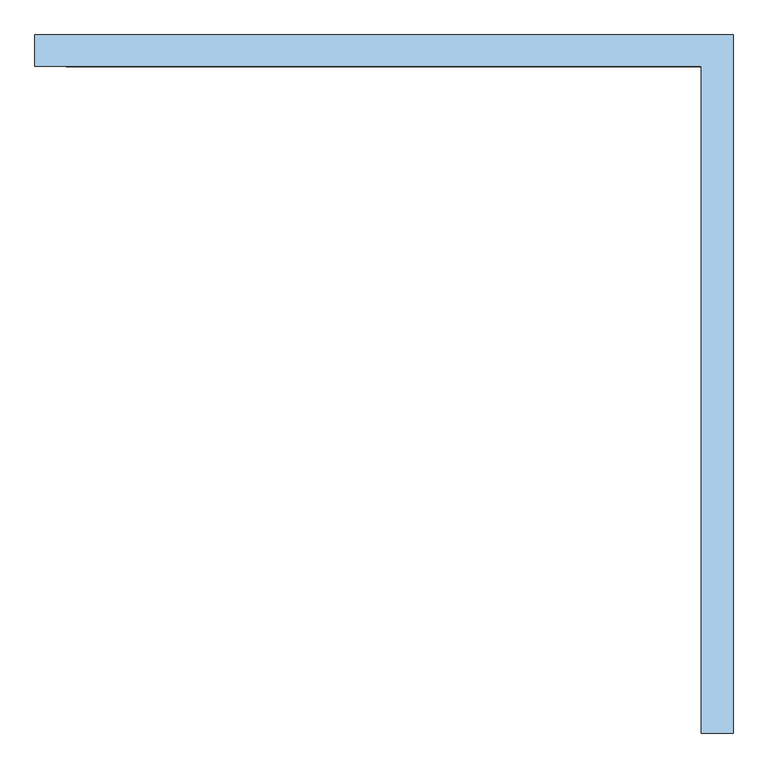
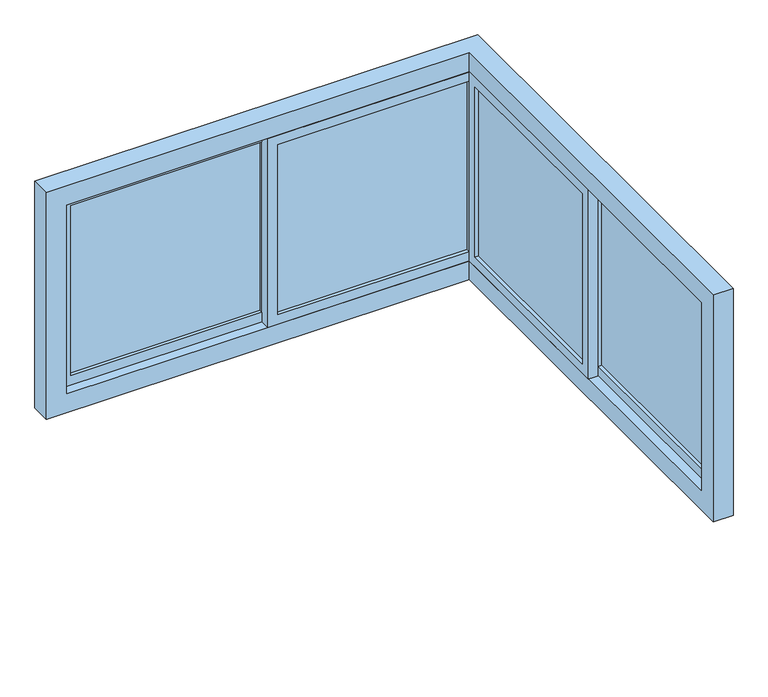
"""IFC4 building model written with IfcOpenShell, lengths in millimetres: window geometry, .CC_ND 300_JANELA DE CANTO_4 FOLHAS DE CORRER_VIDRO : 1.20F X 1.20E X 0.60H."""

import ifcopenshell
import ifcopenshell.guid

model = None  # the IFC model being written
_history = None  # IfcOwnerHistory: only IFC2X3 demands one
_inside = {}  # id of a spatial element -> (the spatial element, [elements in it])
_under = {}  # id of a project, library or spatial element -> (it, [spatial elements below it])
_declared = {}  # id of a project -> (the project, [libraries it declares])
_typed = {}  # id of a type object -> (the type object, [elements of that type])
_made_of = {}  # id of a material, layer set ... -> (it, [elements and type objects made of it])


def new_model(schema):
    """Start an empty IFC model of exactly this schema.

    Asked for "IFC4X3", IfcOpenShell would pick the latest addendum, in which some entities
    have other attributes; the version numbers below select the first issue.
    IFC2X3 requires an IfcOwnerHistory on every rooted entity: one is made here for all.
    """
    global model, _history
    if schema == "IFC4X3":
        model = ifcopenshell.file(schema_version=(4, 3, 0, 0))
    else:
        model = ifcopenshell.file(schema=schema)
    _inside.clear()
    _under.clear()
    _declared.clear()
    _typed.clear()
    _made_of.clear()
    _history = None
    if model.schema == "IFC2X3":
        org = make("IfcOrganization", Name="unknown")
        user = make(
            "IfcPersonAndOrganization",
            ThePerson=make("IfcPerson", FamilyName="unknown"),
            TheOrganization=org,
        )
        app = make(
            "IfcApplication",
            ApplicationDeveloper=org,
            Version="unknown",
            ApplicationFullName="unknown",
            ApplicationIdentifier="unknown",
        )
        _history = make(
            "IfcOwnerHistory",
            OwningUser=user,
            OwningApplication=app,
            ChangeAction="ADDED",
            CreationDate=0,
        )
    return model


def make(cls, **values):
    """One entity of the class cls with the attributes given. An attribute that is None is left unset."""
    return model.create_entity(
        cls, **{name: value for name, value in values.items() if value is not None}
    )


def rooted(cls, **values):
    """An entity with a GlobalId (a new one), such as an element, a storey or a relation."""
    return make(cls, GlobalId=ifcopenshell.guid.new(), OwnerHistory=_history, **values)


def si_unit(unit_type, name, prefix=None):
    """IfcSIUnit, for example si_unit("LENGTHUNIT", "METRE", prefix="MILLI")."""
    return make("IfcSIUnit", UnitType=unit_type, Prefix=prefix, Name=name)


def assignment(units):
    """IfcUnitAssignment: the units of a project."""
    return None if units is None else make("IfcUnitAssignment", Units=units)


def point(xyz):
    """IfcCartesianPoint."""
    return None if xyz is None else make("IfcCartesianPoint", Coordinates=xyz)


def direction(xyz):
    """IfcDirection."""
    return None if xyz is None else make("IfcDirection", DirectionRatios=xyz)


def frame(location, z_axis=None, x_axis=None):
    """IfcAxis2Placement3D, a coordinate frame: its origin and axes. An axis left out is left unset."""
    return make(
        "IfcAxis2Placement3D",
        Location=point(location),
        Axis=direction(z_axis),
        RefDirection=direction(x_axis),
    )


def origin():
    """The frame at (0, 0, 0) with its axes left unset."""
    return frame((0.0, 0.0, 0.0))


def place(relative_to, where):
    """IfcLocalPlacement: puts the frame where relative to a parent placement (None: the world)."""
    return make(
        "IfcLocalPlacement", PlacementRelTo=relative_to, RelativePlacement=where
    )


def context(
    kind, dimensions, precision=None, world=None, true_north=None, identifier=None
):
    """IfcGeometricRepresentationContext, for example the 3D "Model" context."""
    return make(
        "IfcGeometricRepresentationContext",
        ContextIdentifier=identifier,
        ContextType=kind,
        CoordinateSpaceDimension=dimensions,
        Precision=precision,
        WorldCoordinateSystem=world,
        TrueNorth=true_north,
    )


def project(units=None, contexts=None):
    """IfcProject with its units and contexts."""
    return rooted(
        "IfcProject",
        Name="project",
        RepresentationContexts=contexts,
        UnitsInContext=assignment(units),
    )


def spatial(cls, under=None, at=None, **own):
    """A site, building, storey or space (cls), placed at a placement, below another one or the project."""
    s = rooted(cls, ObjectPlacement=at, **own)
    if under is not None:
        _under.setdefault(under.id(), (under, []))[1].append(s)
    return s


def polyline(points):
    """IfcPolyline through the points."""
    return make("IfcPolyline", Points=[point(p) for p in points])


def outline(outer, holes=None, kind="AREA"):
    """IfcArbitraryClosedProfileDef: a profile drawn as a closed curve; with holes, ...WithVoids."""
    if holes is None:
        return make("IfcArbitraryClosedProfileDef", ProfileType=kind, OuterCurve=outer)
    return make(
        "IfcArbitraryProfileDefWithVoids",
        ProfileType=kind,
        OuterCurve=outer,
        InnerCurves=holes,
    )


def extrude(swept, where, along, depth):
    """IfcExtrudedAreaSolid: the profile swept, set in the frame where, extruded along a direction by depth."""
    return make(
        "IfcExtrudedAreaSolid",
        SweptArea=swept,
        Position=where,
        ExtrudedDirection=direction(along),
        Depth=depth,
    )


def faces_of(points, faces, orient=None, outer=None):
    """IfcFace entities. A face is a list of loops; a loop is a list of indices into points, from 0.

    orient and outer hold one flag for each loop. By default every Orientation is true, the
    first loop of a face is its IfcFaceOuterBound and the others are IfcFaceBound.
    """
    made = []
    for i, loops in enumerate(faces):
        bounds = []
        for j, loop in enumerate(loops):
            is_outer = j == 0 if outer is None else outer[i][j]
            bounds.append(
                make(
                    "IfcFaceOuterBound" if is_outer else "IfcFaceBound",
                    Bound=make("IfcPolyLoop", Polygon=[points[k] for k in loop]),
                    Orientation=True if orient is None else orient[i][j],
                )
            )
        made.append(make("IfcFace", Bounds=bounds))
    return made


def faceted_brep(points, faces, orient=None, outer=None, voids=None):
    """IfcFacetedBrep: a solid bounded by flat faces; with voids (closed shells), ...WithVoids."""
    shared = [point(p) for p in points]
    hull = make("IfcClosedShell", CfsFaces=faces_of(shared, faces, orient, outer))
    if voids is None:
        return make("IfcFacetedBrep", Outer=hull)
    return make(
        "IfcFacetedBrepWithVoids",
        Outer=hull,
        Voids=[
            make(cls, CfsFaces=faces_of(shared, fs, o, b)) for cls, fs, o, b in voids
        ],
    )


def shape(context_of_items, identifier, shape_type, items):
    """IfcShapeRepresentation: the items that make up one representation, for example the "Body"."""
    return make(
        "IfcShapeRepresentation",
        ContextOfItems=context_of_items,
        RepresentationIdentifier=identifier,
        RepresentationType=shape_type,
        Items=items,
    )


def source(mapping_origin, context_of_items, identifier, shape_type, items):
    """IfcRepresentationMap: a shape defined once, which mapped items show again and again."""
    return make(
        "IfcRepresentationMap",
        MappingOrigin=mapping_origin,
        MappedRepresentation=shape(context_of_items, identifier, shape_type, items),
    )


def transform(
    local_origin,
    x_axis=None,
    y_axis=None,
    z_axis=None,
    scale=None,
    scale2=None,
    scale3=None,
    uniform=True,
):
    """IfcCartesianTransformationOperator3D, or its non-uniform kind. x_axis, y_axis, z_axis: its Axis1, 2, 3."""
    if uniform:
        return make(
            "IfcCartesianTransformationOperator3D",
            Axis1=direction(x_axis),
            Axis2=direction(y_axis),
            LocalOrigin=point(local_origin),
            Scale=scale,
            Axis3=direction(z_axis),
        )
    return make(
        "IfcCartesianTransformationOperator3DnonUniform",
        Axis1=direction(x_axis),
        Axis2=direction(y_axis),
        LocalOrigin=point(local_origin),
        Scale=scale,
        Axis3=direction(z_axis),
        Scale2=scale2,
        Scale3=scale3,
    )


def mapped(mapping_source, mapping_target):
    """IfcMappedItem: shows the shape of a source again, moved by a transform."""
    return make(
        "IfcMappedItem", MappingSource=mapping_source, MappingTarget=mapping_target
    )


def made_of(thing, what):
    """Note that an element or type object is made of a material, layer set ...; save() writes the relation."""
    if what is not None:
        _made_of.setdefault(what.id(), (what, []))[1].append(thing)
    return thing


def element(
    cls,
    number,
    at=None,
    inside=None,
    cuts=None,
    type_object=None,
    material=None,
    context=None,
    identifier="Body",
    shape_type=None,
    held_by="IfcProductDefinitionShape",
    body=None,
    shapes=None,
    **own,
):
    """One element of the class cls, such as IfcWall. Its Tag is "e" and its number.

    at: its placement. inside: the storey or other place that contains it. cuts: it is an
    opening in that element (IfcRelVoidsElement). A single representation is given by context,
    identifier, shape_type and body (its items); several are given by shapes. held_by: the class
    of the entity that holds the representations. save() writes the other relations.
    """
    e = rooted(cls, Tag="e%d" % number, ObjectPlacement=at, **own)
    if body is not None:
        shapes = [shape(context, identifier, shape_type, body)]
    if shapes is not None:
        e.Representation = make(held_by, Representations=shapes)
    if inside is not None:
        _inside.setdefault(inside.id(), (inside, []))[1].append(e)
    if cuts is not None:
        rooted(
            "IfcRelVoidsElement", RelatingBuildingElement=cuts, RelatedOpeningElement=e
        )
    if type_object is not None:
        _typed.setdefault(type_object.id(), (type_object, []))[1].append(e)
    return made_of(e, material)


def aggregate(whole, parts):
    """IfcRelAggregates: a whole, such as a stair, and the parts it consists of."""
    return rooted("IfcRelAggregates", RelatingObject=whole, RelatedObjects=parts)


def save(model, path):
    """Write the relations noted so far, then the file.

    IfcRelAggregates (storeys below a building ...), IfcRelContainedInSpatialStructure (elements
    in a storey), IfcRelDefinesByType, IfcRelAssociatesMaterial and IfcRelDeclares: one each for
    every whole, place, type object, material and project.
    """
    for whole, parts in _under.values():
        aggregate(whole, parts)
    for where, things in _inside.values():
        rooted(
            "IfcRelContainedInSpatialStructure",
            RelatedElements=things,
            RelatingStructure=where,
        )
    for kind, things in _typed.values():
        rooted("IfcRelDefinesByType", RelatedObjects=things, RelatingType=kind)
    for what, things in _made_of.values():
        rooted("IfcRelAssociatesMaterial", RelatedObjects=things, RelatingMaterial=what)
    for by, libraries in _declared.values():
        rooted("IfcRelDeclares", RelatingContext=by, RelatedDefinitions=libraries)
    model.write(path)


def window_65d6727e(model_context):
    return source(origin(), model_context, "Body", "SolidModel", [
        extrude(outline(polyline([(-516.0, 1950.0), (-516.0, 1450.0), (-1032.0, 1450.0), (-1032.0, 1950.0), (-516.0, 1950.0)]), holes=[polyline([(-541.0, 1925.0), (-1007.0, 1925.0), (-1007.0, 1475.0), (-541.0, 1475.0), (-541.0, 1925.0)])]), frame((482.0, 0.0, 0.0), z_axis=(1.0, 0.0, 0.0), x_axis=(0.0, 1.0, 0.0)), (0.0, 0.0, 1.0), 25.0),
        extrude(outline(polyline([(490.5, -541.0), (498.5, -541.0), (498.5, -1007.0), (490.5, -1007.0), (490.5, -541.0)])), frame((0.0, 0.0, 1475.0), z_axis=(0.0, 0.0, 1.0), x_axis=(1.0, 0.0, 0.0)), (0.0, 0.0, 1.0), 450.0),
        extrude(outline(polyline([(-25.0, 1950.0), (-25.0, 1450.0), (-541.0, 1450.0), (-541.0, 1950.0), (-25.0, 1950.0)]), holes=[polyline([(-50.0, 1925.0), (-516.0, 1925.0), (-516.0, 1475.0), (-50.0, 1475.0), (-50.0, 1925.0)])]), frame((457.0, 0.0, 0.0), z_axis=(1.0, 0.0, 0.0), x_axis=(0.0, 1.0, 0.0)), (0.0, 0.0, 1.0), 25.0),
        extrude(outline(polyline([(465.5, -50.0), (473.5, -50.0), (473.5, -516.0), (465.5, -516.0), (465.5, -50.0)])), frame((0.0, 0.0, 1475.0), z_axis=(0.0, 0.0, 1.0), x_axis=(1.0, 0.0, 0.0)), (0.0, 0.0, 1.0), 450.0),
        extrude(outline(polyline([(1950.0, 482.0), (1950.0, -46.5), (1450.0, -46.5), (1450.0, 482.0), (1950.0, 482.0)]), holes=[polyline([(1925.0, 457.0), (1475.0, 457.0), (1475.0, -21.5), (1925.0, -21.5), (1925.0, 457.0)])]), frame((0.0, -25.0, 0.0), z_axis=(0.0, 1.0, 0.0), x_axis=(0.0, 0.0, 1.0)), (0.0, 0.0, 1.0), 25.0),
        extrude(outline(polyline([(457.0, -8.5), (457.0, -16.5), (-21.5, -16.5), (-21.5, -8.5), (457.0, -8.5)])), frame((0.0, 0.0, 1475.0), z_axis=(0.0, 0.0, 1.0), x_axis=(1.0, 0.0, 0.0)), (0.0, 0.0, 1.0), 450.0),
        extrude(outline(polyline([(1950.0, -21.5), (1950.0, -550.0), (1450.0, -550.0), (1450.0, -21.5), (1950.0, -21.5)]), holes=[polyline([(1925.0, -46.5), (1475.0, -46.5), (1475.0, -525.0), (1925.0, -525.0), (1925.0, -46.5)])]), frame((0.0, 0.0, 0.0), z_axis=(0.0, 1.0, 0.0), x_axis=(0.0, 0.0, 1.0)), (0.0, 0.0, 1.0), 25.0),
        extrude(outline(polyline([(-46.5, 16.5), (-46.5, 8.5), (-525.0, 8.5), (-525.0, 16.5), (-46.5, 16.5)])), frame((0.0, 0.0, 1475.0), z_axis=(0.0, 0.0, 1.0), x_axis=(1.0, 0.0, 0.0)), (0.0, 0.0, 1.0), 450.0),
        faceted_brep([(457.0, -1082.0, 1400.0), (457.0, -1082.0, 2000.0), (457.0, -25.0, 2000.0), (457.0, -25.0, 1950.0), (457.0, -1032.0, 1950.0), (457.0, -1032.0, 1450.0), (457.0, -25.0, 1450.0), (457.0, -25.0, 1400.0), (507.0, -1082.0, 1400.0), (507.0, -1082.0, 2000.0), (507.0, -1032.0, 1950.0), (507.0, -1032.0, 1450.0), (507.0, 25.0, 1450.0), (-550.0, 25.0, 1450.0), (-550.0, -25.0, 1450.0), (-600.0, -25.0, 2000.0), (-600.0, -25.0, 1400.0), (-550.0, -25.0, 1950.0), (507.0, 25.0, 1400.0), (-600.0, 25.0, 1400.0), (507.0, 25.0, 1950.0), (507.0, 25.0, 2000.0), (-550.0, 25.0, 1950.0), (-600.0, 25.0, 2000.0)], [[[0, 1, 2, 3, 4, 5, 6, 7]], [[1, 0, 8, 9]], [[5, 4, 10, 11]], [[5, 11, 12, 13, 14, 6]], [[15, 16, 7, 6, 14, 17, 3, 2]], [[18, 8, 0, 7, 16, 19]], [[12, 11, 10, 20, 21, 9, 8, 18]], [[21, 20, 22, 13, 12, 18, 19, 23]], [[17, 14, 13, 22]], [[16, 15, 23, 19]], [[20, 10, 4, 3, 17, 22]], [[1, 9, 21, 23, 15, 2]]]),
    ])


if __name__ == "__main__":
    model = new_model("IFC4")
    model_context = context("Model", 3, world=origin())
    ifc_project = project(units=[si_unit("LENGTHUNIT", "METRE", prefix="MILLI")], contexts=[model_context])
    site = spatial("IfcSite", under=ifc_project)
    building = spatial("IfcBuilding", under=site)
    placement = place(None, origin())
    window_shape = window_65d6727e(model_context)
    element("IfcWindow", 1, ObjectType=".CC_ND 300_JANELA DE CANTO_4 FOLHAS DE CORRER_VIDRO : 1.20F X 1.20E X 0.60H", at=placement, inside=building, context=model_context, shape_type="MappedRepresentation", body=[
        mapped(window_shape, transform((0.0, 0.0, 0.0), x_axis=(1.0, 0.0, 0.0), y_axis=(0.0, 1.0, 0.0), z_axis=(0.0, 0.0, 1.0))),
    ])
    save(model, "model.ifc")

# Revit data of these elements
# Type ".CC_ND 300_JANELA DE CANTO_4 FOLHAS DE CORRER_VIDRO : 1.20F X 1.20E X 0.60H"
#   Type Mark = "57"
#   Vidro_Espessura [instance default] = 0.008 m
#   Painéis_Altura [instance default] = 0.50 m
#   Moldura Painéis_Espessura [instance default] = 0.025 m
#   Moldura Janela_Largura [instance default] = 0.05 m
#   Painéis Frente_Largura [instance default] = 0.5375 m
#   Painéis Esquerda_Largura [instance default] = 0.525 m
#   Moldura Janela_Extensão Interior [instance default] = 0.025 m
#   Moldura Janela_Extensão Frente [instance default] = 0.025 m
#   Rough Width = 2.40 m
#   Largura Frontal = 1.20 m
#   Largura Esquerda = 1.20 m
#   Moldura Painéis_Largura [instance default] = 0.025 m
#   Espessura da parede [instance default] = 0.20 m
#   Moldura Janela_Espessura [instance default] = 0.05 m
#   Height = 0.60 m
#   Altura-padrão do peitoril [instance default] = 1.40 m
#   Width = 2.40 m
#   Vidro [instance default] = none
#   Moldura/Painéis [instance default] = none
#   Rough Height = 0
#   Wall Closure = (empty or 0)
# Element 1 (IfcWindow, ".CC_ND 300_JANELA DE CANTO_4 FOLHAS DE CORRER_VIDRO : 1.20F X 1.20E X 0.60H")
#   Painéis Frente_Largura = 0.5285 m
#   Painéis Esquerda_Largura = 0.516 m
#   Espessura da parede = 0.236 m
#   Vidro = .VIDRO GENÉRICO
#   Moldura/Painéis = .ALUMÍNIO COM PINTURA ELETROSTÁTICA BRANCA
#   Materials on its faces: ".ALUMÍNIO COM PINTURA ELETROSTÁTICA BRANCA", ".VIDRO GENÉRICO"
# Materials
#   ".ALUMÍNIO COM PINTURA ELETROSTÁTICA BRANCA": class "CC_METAIS", colour RGB 241 241 241, transparency 0, Cost = 0
#   ".VIDRO GENÉRICO": class ".CC_VIDRO", colour RGB 0 128 192, transparency 0.9, Description = "Vidro comum", Cost = 0
